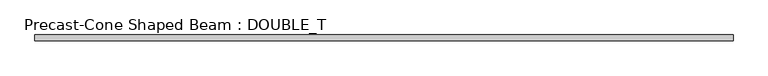
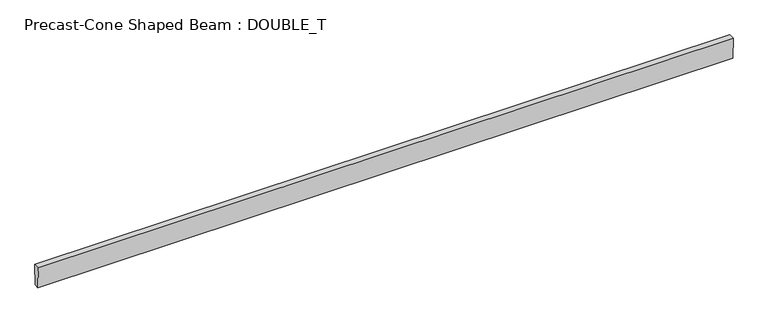
"""IFC4 building model written with IfcOpenShell, lengths in millimetres: beam geometry, Precast-Cone Shaped Beam : DOUBLE_T."""

import ifcopenshell
import ifcopenshell.guid

model = None  # the IFC model being written
_history = None  # IfcOwnerHistory: only IFC2X3 demands one
_inside = {}  # id of a spatial element -> (the spatial element, [elements in it])
_under = {}  # id of a project, library or spatial element -> (it, [spatial elements below it])
_declared = {}  # id of a project -> (the project, [libraries it declares])
_typed = {}  # id of a type object -> (the type object, [elements of that type])
_made_of = {}  # id of a material, layer set ... -> (it, [elements and type objects made of it])


def new_model(schema):
    """Start an empty IFC model of exactly this schema.

    Asked for "IFC4X3", IfcOpenShell would pick the latest addendum, in which some entities
    have other attributes; the version numbers below select the first issue.
    IFC2X3 requires an IfcOwnerHistory on every rooted entity: one is made here for all.
    """
    global model, _history
    if schema == "IFC4X3":
        model = ifcopenshell.file(schema_version=(4, 3, 0, 0))
    else:
        model = ifcopenshell.file(schema=schema)
    _inside.clear()
    _under.clear()
    _declared.clear()
    _typed.clear()
    _made_of.clear()
    _history = None
    if model.schema == "IFC2X3":
        org = make("IfcOrganization", Name="unknown")
        user = make(
            "IfcPersonAndOrganization",
            ThePerson=make("IfcPerson", FamilyName="unknown"),
            TheOrganization=org,
        )
        app = make(
            "IfcApplication",
            ApplicationDeveloper=org,
            Version="unknown",
            ApplicationFullName="unknown",
            ApplicationIdentifier="unknown",
        )
        _history = make(
            "IfcOwnerHistory",
            OwningUser=user,
            OwningApplication=app,
            ChangeAction="ADDED",
            CreationDate=0,
        )
    return model


def make(cls, **values):
    """One entity of the class cls with the attributes given. An attribute that is None is left unset."""
    return model.create_entity(
        cls, **{name: value for name, value in values.items() if value is not None}
    )


def rooted(cls, **values):
    """An entity with a GlobalId (a new one), such as an element, a storey or a relation."""
    return make(cls, GlobalId=ifcopenshell.guid.new(), OwnerHistory=_history, **values)


def si_unit(unit_type, name, prefix=None):
    """IfcSIUnit, for example si_unit("LENGTHUNIT", "METRE", prefix="MILLI")."""
    return make("IfcSIUnit", UnitType=unit_type, Prefix=prefix, Name=name)


def assignment(units):
    """IfcUnitAssignment: the units of a project."""
    return None if units is None else make("IfcUnitAssignment", Units=units)


def point(xyz):
    """IfcCartesianPoint."""
    return None if xyz is None else make("IfcCartesianPoint", Coordinates=xyz)


def direction(xyz):
    """IfcDirection."""
    return None if xyz is None else make("IfcDirection", DirectionRatios=xyz)


def frame(location, z_axis=None, x_axis=None):
    """IfcAxis2Placement3D, a coordinate frame: its origin and axes. An axis left out is left unset."""
    return make(
        "IfcAxis2Placement3D",
        Location=point(location),
        Axis=direction(z_axis),
        RefDirection=direction(x_axis),
    )


def origin():
    """The frame at (0, 0, 0) with its axes left unset."""
    return frame((0.0, 0.0, 0.0))


def place(relative_to, where):
    """IfcLocalPlacement: puts the frame where relative to a parent placement (None: the world)."""
    return make(
        "IfcLocalPlacement", PlacementRelTo=relative_to, RelativePlacement=where
    )


def context(
    kind, dimensions, precision=None, world=None, true_north=None, identifier=None
):
    """IfcGeometricRepresentationContext, for example the 3D "Model" context."""
    return make(
        "IfcGeometricRepresentationContext",
        ContextIdentifier=identifier,
        ContextType=kind,
        CoordinateSpaceDimension=dimensions,
        Precision=precision,
        WorldCoordinateSystem=world,
        TrueNorth=true_north,
    )


def project(units=None, contexts=None):
    """IfcProject with its units and contexts."""
    return rooted(
        "IfcProject",
        Name="project",
        RepresentationContexts=contexts,
        UnitsInContext=assignment(units),
    )


def spatial(cls, under=None, at=None, **own):
    """A site, building, storey or space (cls), placed at a placement, below another one or the project."""
    s = rooted(cls, ObjectPlacement=at, **own)
    if under is not None:
        _under.setdefault(under.id(), (under, []))[1].append(s)
    return s


def polyline(points):
    """IfcPolyline through the points."""
    return make("IfcPolyline", Points=[point(p) for p in points])


def outline(outer, holes=None, kind="AREA"):
    """IfcArbitraryClosedProfileDef: a profile drawn as a closed curve; with holes, ...WithVoids."""
    if holes is None:
        return make("IfcArbitraryClosedProfileDef", ProfileType=kind, OuterCurve=outer)
    return make(
        "IfcArbitraryProfileDefWithVoids",
        ProfileType=kind,
        OuterCurve=outer,
        InnerCurves=holes,
    )


def extrude(swept, where, along, depth):
    """IfcExtrudedAreaSolid: the profile swept, set in the frame where, extruded along a direction by depth."""
    return make(
        "IfcExtrudedAreaSolid",
        SweptArea=swept,
        Position=where,
        ExtrudedDirection=direction(along),
        Depth=depth,
    )


def shape(context_of_items, identifier, shape_type, items):
    """IfcShapeRepresentation: the items that make up one representation, for example the "Body"."""
    return make(
        "IfcShapeRepresentation",
        ContextOfItems=context_of_items,
        RepresentationIdentifier=identifier,
        RepresentationType=shape_type,
        Items=items,
    )


def source(mapping_origin, context_of_items, identifier, shape_type, items):
    """IfcRepresentationMap: a shape defined once, which mapped items show again and again."""
    return make(
        "IfcRepresentationMap",
        MappingOrigin=mapping_origin,
        MappedRepresentation=shape(context_of_items, identifier, shape_type, items),
    )


def transform(
    local_origin,
    x_axis=None,
    y_axis=None,
    z_axis=None,
    scale=None,
    scale2=None,
    scale3=None,
    uniform=True,
):
    """IfcCartesianTransformationOperator3D, or its non-uniform kind. x_axis, y_axis, z_axis: its Axis1, 2, 3."""
    if uniform:
        return make(
            "IfcCartesianTransformationOperator3D",
            Axis1=direction(x_axis),
            Axis2=direction(y_axis),
            LocalOrigin=point(local_origin),
            Scale=scale,
            Axis3=direction(z_axis),
        )
    return make(
        "IfcCartesianTransformationOperator3DnonUniform",
        Axis1=direction(x_axis),
        Axis2=direction(y_axis),
        LocalOrigin=point(local_origin),
        Scale=scale,
        Axis3=direction(z_axis),
        Scale2=scale2,
        Scale3=scale3,
    )


def mapped(mapping_source, mapping_target):
    """IfcMappedItem: shows the shape of a source again, moved by a transform."""
    return make(
        "IfcMappedItem", MappingSource=mapping_source, MappingTarget=mapping_target
    )


def made_of(thing, what):
    """Note that an element or type object is made of a material, layer set ...; save() writes the relation."""
    if what is not None:
        _made_of.setdefault(what.id(), (what, []))[1].append(thing)
    return thing


def element(
    cls,
    number,
    at=None,
    inside=None,
    cuts=None,
    type_object=None,
    material=None,
    context=None,
    identifier="Body",
    shape_type=None,
    held_by="IfcProductDefinitionShape",
    body=None,
    shapes=None,
    **own,
):
    """One element of the class cls, such as IfcWall. Its Tag is "e" and its number.

    at: its placement. inside: the storey or other place that contains it. cuts: it is an
    opening in that element (IfcRelVoidsElement). A single representation is given by context,
    identifier, shape_type and body (its items); several are given by shapes. held_by: the class
    of the entity that holds the representations. save() writes the other relations.
    """
    e = rooted(cls, Tag="e%d" % number, ObjectPlacement=at, **own)
    if body is not None:
        shapes = [shape(context, identifier, shape_type, body)]
    if shapes is not None:
        e.Representation = make(held_by, Representations=shapes)
    if inside is not None:
        _inside.setdefault(inside.id(), (inside, []))[1].append(e)
    if cuts is not None:
        rooted(
            "IfcRelVoidsElement", RelatingBuildingElement=cuts, RelatedOpeningElement=e
        )
    if type_object is not None:
        _typed.setdefault(type_object.id(), (type_object, []))[1].append(e)
    return made_of(e, material)


def aggregate(whole, parts):
    """IfcRelAggregates: a whole, such as a stair, and the parts it consists of."""
    return rooted("IfcRelAggregates", RelatingObject=whole, RelatedObjects=parts)


def save(model, path):
    """Write the relations noted so far, then the file.

    IfcRelAggregates (storeys below a building ...), IfcRelContainedInSpatialStructure (elements
    in a storey), IfcRelDefinesByType, IfcRelAssociatesMaterial and IfcRelDeclares: one each for
    every whole, place, type object, material and project.
    """
    for whole, parts in _under.values():
        aggregate(whole, parts)
    for where, things in _inside.values():
        rooted(
            "IfcRelContainedInSpatialStructure",
            RelatedElements=things,
            RelatingStructure=where,
        )
    for kind, things in _typed.values():
        rooted("IfcRelDefinesByType", RelatedObjects=things, RelatingType=kind)
    for what, things in _made_of.values():
        rooted("IfcRelAssociatesMaterial", RelatedObjects=things, RelatingMaterial=what)
    for by, libraries in _declared.values():
        rooted("IfcRelDeclares", RelatingContext=by, RelatedDefinitions=libraries)
    model.write(path)


def precast_cone_shaped_beam_double_t_17914b82(model_context):
    return source(origin(), model_context, "Body", "SweptSolid", [
        extrude(outline(polyline([(-50.8, -228.6), (-63.5, 228.6), (63.5, 228.6), (50.8, -228.6), (-50.8, -228.6)])), frame((-7594.6, 0.0, 0.0), z_axis=(1.0, 0.0, 0.0), x_axis=(0.0, 1.0, 0.0)), (0.0, 0.0, 1.0), 14973.3),
    ])


if __name__ == "__main__":
    model = new_model("IFC4")
    model_context = context("Model", 3, world=origin())
    ifc_project = project(units=[si_unit("LENGTHUNIT", "METRE", prefix="MILLI")], contexts=[model_context])
    site = spatial("IfcSite", under=ifc_project)
    building = spatial("IfcBuilding", under=site)
    placement = place(None, origin())
    precast_cone_shaped_beam_double_t_shape = precast_cone_shaped_beam_double_t_17914b82(model_context)
    element("IfcBeam", 1, ObjectType="Precast-Cone Shaped Beam : DOUBLE_T", at=placement, inside=building, context=model_context, shape_type="MappedRepresentation", body=[
        mapped(precast_cone_shaped_beam_double_t_shape, transform((0.0, 0.0, 0.0), x_axis=(1.0, 0.0, 0.0), y_axis=(0.0, 1.0, 0.0), z_axis=(0.0, 0.0, 1.0))),
    ])
    save(model, "model.ifc")

# Revit data of these elements
# Type "Precast-Cone Shaped Beam : DOUBLE_T"
#   Top Width = 0' - 5"
#   Tie Rod Weight [instance default] = 30
#   Tie Rod W [instance default] = 0.0660938 kip
#   Single Rebar Weight [instance default] = 50
#   Single Rebar W [instance default] = 0.110156 kip
#   Rebar Grids Weight [instance default] = 100
#   Rebar Grids W [instance default] = 0.220313 kip
#   Depth = 1' - 6"
#   Bottom Width = 0' - 4"
#   Length [instance default] = 5' - 0"
#   Structural Material [instance default] = Concrete, Precast
#   Assembly Code = ""
# Element 1 (IfcBeam, "Precast-Cone Shaped Beam : DOUBLE_T")
#   Length = 49' - 6"
#   Structural Material = Concrete - Precast Concrete - Normal Weight Concrete - 5 ksi
#   Materials on its faces: "Concrete - Precast Concrete - Normal Weight Concrete - 5 ksi"
# Materials
#   "Concrete, Precast": class "Concrete", colour RGB 198 187 187, transparency 0, Description = "Precast concrete", Cost = 0
#   "Concrete - Precast Concrete - Normal Weight Concrete - 5 ksi": class "Concrete", colour RGB 198 187 187, transparency 0, Cost = 0
